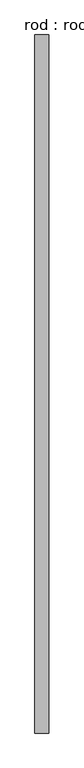
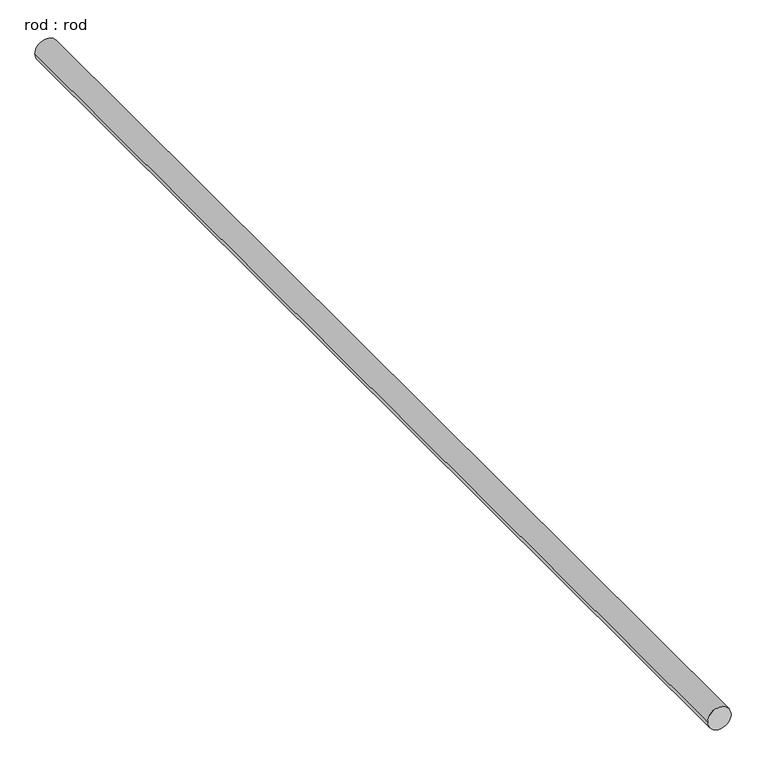
"""IFC4 building model written with IfcOpenShell, lengths in millimetres: proxy geometry, rod : rod."""

from ifc_helpers import new_model, si_unit, point, frame, frame_2d, origin, place, context, project, spatial, circle_curve, trimmed, segment, composite_curve, outline, extrude, source, transform, mapped, element, save


def rod_rod_f9bd0e5a(model_context):
    return source(origin(), model_context, "Body", "SweptSolid", [
        extrude(outline(composite_curve([segment(trimmed(circle_curve(frame_2d((0.0108462, 0.0)), 200.0), [point((0.0108462, 200.0))], [point((0.0108462, -200.0))], False, "CARTESIAN"), True, "CONTINUOUS"), segment(trimmed(circle_curve(frame_2d((0.0108462, 0.0)), 200.0), [point((0.0108462, -200.0))], [point((0.0108462, 200.0))], False, "CARTESIAN"), True, "CONTINUOUS")], self_intersect=False)), frame((0.0, -5857.2713847, 0.0), z_axis=(0.0, 1.0, 0.0), x_axis=(0.0, 0.0, 1.0)), (0.0, 0.0, 1.0), 19900.0),
    ])


if __name__ == "__main__":
    model = new_model("IFC4")
    model_context = context("Model", 3, world=origin())
    ifc_project = project(units=[si_unit("LENGTHUNIT", "METRE", prefix="MILLI")], contexts=[model_context])
    site = spatial("IfcSite", under=ifc_project)
    building = spatial("IfcBuilding", under=site)
    placement = place(None, origin())
    rod_rod_shape = rod_rod_f9bd0e5a(model_context)
    element("IfcBuildingElementProxy", 1, Name="rod : rod", ObjectType="rod : rod", at=placement, inside=building, context=model_context, shape_type="MappedRepresentation", body=[
        mapped(rod_rod_shape, transform((0.0, 0.0, 0.0), x_axis=(1.0, 0.0, 0.0), y_axis=(0.0, 1.0, 0.0), z_axis=(0.0, 0.0, 1.0))),
    ])
    save(model, "model.ifc")

# Revit data of these elements
# Type "rod : rod"
#   Default Elevation = 0
